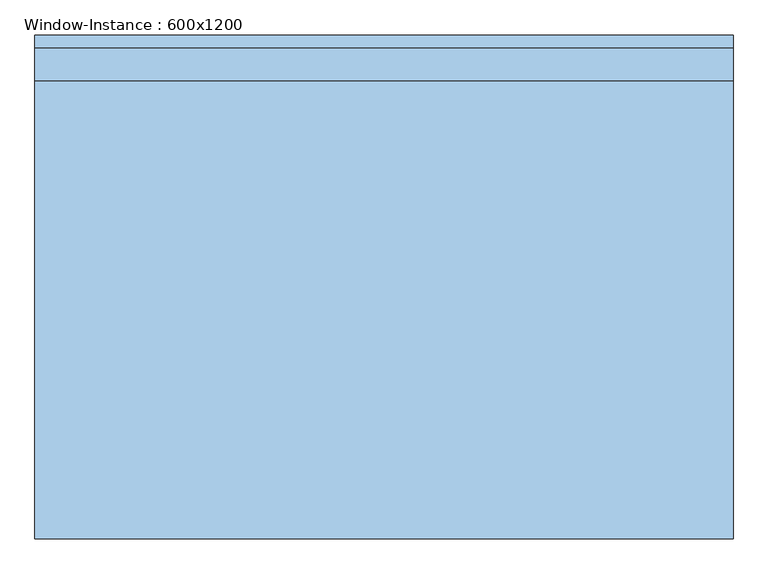
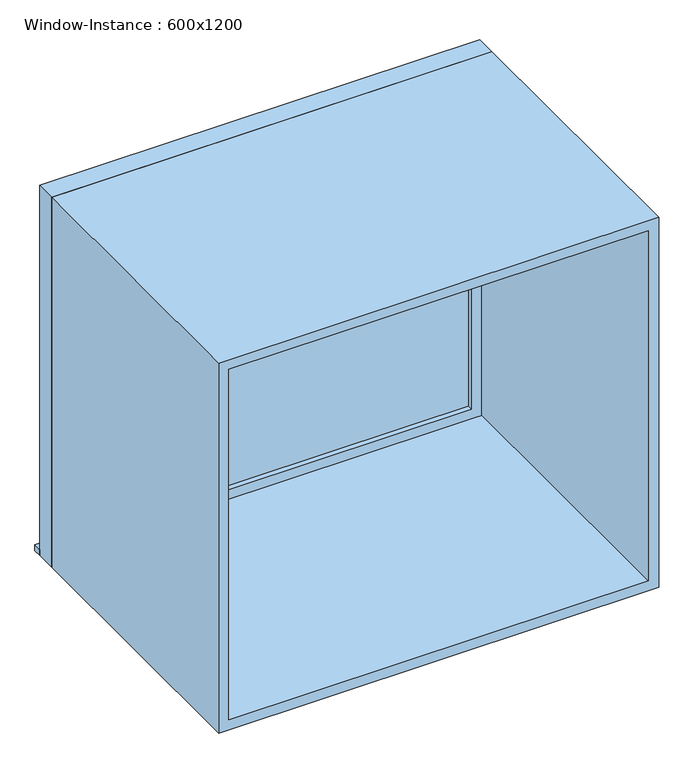
"""IFC4 building model written with IfcOpenShell, lengths in millimetres: window geometry, Window-Instance : 600x1200."""

from ifc_helpers import new_model, si_unit, frame, origin, place, context, project, spatial, polyline, outline, extrude, source, transform, mapped, element, save


def window_instance_600x1200_ff6d469b(model_context):
    return source(origin(), model_context, "Body", "SweptSolid", [
        extrude(outline(polyline([(-713.1, 500.4), (636.9, 500.4), (636.9, 475.0), (-713.1, 475.0), (-713.1, 500.4)])), frame((0.0, 0.0, 900.0), z_axis=(0.0, 0.0, 1.0), x_axis=(1.0, 0.0, 0.0)), (0.0, 0.0, 1.0), 19.05),
        extrude(outline(polyline([(573.4, 426.425), (-649.6, 426.425), (-649.6, 439.125), (573.4, 439.125), (573.4, 426.425)])), frame((0.0, 0.0, 963.5), z_axis=(0.0, 0.0, 1.0), x_axis=(1.0, 0.0, 0.0)), (0.0, 0.0, 1.0), 1073.0),
        extrude(outline(polyline([(2080.95, -694.05), (919.05, -694.05), (919.05, 617.85), (2080.95, 617.85), (2080.95, -694.05)]), holes=[polyline([(2036.5, -649.6), (2036.5, 573.4), (963.5, 573.4), (963.5, -649.6), (2036.5, -649.6)])]), frame((0.0, 410.55, 0.0), z_axis=(0.0, 1.0, 0.0), x_axis=(0.0, 0.0, 1.0)), (0.0, 0.0, 1.0), 44.45),
        extrude(outline(polyline([(2100.0, -713.1), (900.0, -713.1), (900.0, 636.9), (2100.0, 636.9), (2100.0, -713.1)]), holes=[polyline([(2068.25, -681.35), (2068.25, 605.15), (931.75, 605.15), (931.75, -681.35), (2068.25, -681.35)])]), frame((0.0, -475.0, 0.0), z_axis=(0.0, 1.0, 0.0), x_axis=(0.0, 0.0, 1.0)), (0.0, 0.0, 1.0), 885.55),
        extrude(outline(polyline([(2100.0, 636.9), (2100.0, -713.1), (900.0, -713.1), (900.0, 636.9), (2100.0, 636.9)]), holes=[polyline([(2080.95, 617.85), (919.05, 617.85), (919.05, -694.05), (2080.95, -694.05), (2080.95, 617.85)])]), frame((0.0, 410.55, 0.0), z_axis=(0.0, 1.0, 0.0), x_axis=(0.0, 0.0, 1.0)), (0.0, 0.0, 1.0), 64.45),
    ])


if __name__ == "__main__":
    model = new_model("IFC4")
    model_context = context("Model", 3, world=origin())
    ifc_project = project(units=[si_unit("LENGTHUNIT", "METRE", prefix="MILLI")], contexts=[model_context])
    site = spatial("IfcSite", under=ifc_project)
    building = spatial("IfcBuilding", under=site)
    placement = place(None, origin())
    window_instance_600x1200_shape = window_instance_600x1200_ff6d469b(model_context)
    element("IfcWindow", 1, ObjectType="Window-Instance : 600x1200", at=placement, inside=building, context=model_context, shape_type="MappedRepresentation", body=[
        mapped(window_instance_600x1200_shape, transform((0.0, 0.0, 0.0), x_axis=(1.0, 0.0, 0.0), y_axis=(0.0, 1.0, 0.0), z_axis=(0.0, 0.0, 1.0))),
    ])
    save(model, "model.ifc")

# Revit data of these elements
# Type "Window-Instance : 600x1200"
#   Type Mark = "7"
#   Construction Type Id = "GSP4R"
#   Assembly Code = "B2020100"
#   Analytic Construction = "1/8 in Pilkington single glazing"
#   Visual Light Transmittance = 0.9
#   Thermal Resistance (R) = 0.149095 (m²·K)/W
#   Solar Heat Gain Coefficient = 0.86
#   Heat Transfer Coefficient (U) = 6.70716 W/(m²·K)
#   Height [instance default] = 1200 mm
#   Default Sill Height = 900 mm
#   Width [instance default] = 600 mm
#   Window Inset = 20 mm
#   Glass Pane Material = WW-EC-GL-Storefront
#   Sash Material = WW-EC-RGB-White
#   Wall Closure = (empty or 0)
# Element 1 (IfcWindow, "Window-Instance : 600x1200")
#   Width = 1350 mm
#   Materials on its faces: "WW-EC-RGB-White", "WW-EC-GL-Storefront"
# Materials
#   "WW-EC-GL-Storefront": class "Glass", colour RGB 236 240 239, transparency 0.85, Description = "Storefront Glass", Cost = 0
#   "WW-EC-RGB-White": class "Generic", colour RGB 255 255 255, transparency 0, Comments = "If region requests off-white, swith asset color to RGB 231-228-220", Description = "Generic Color", Cost = 0
